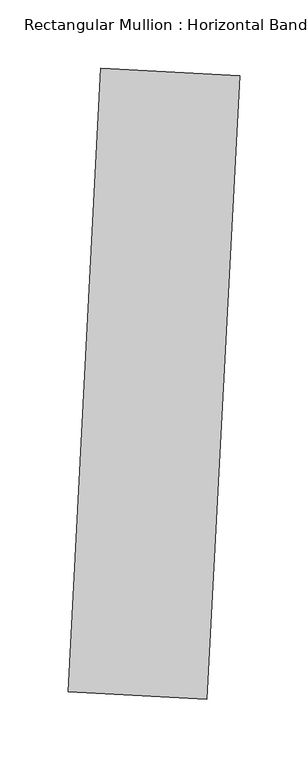
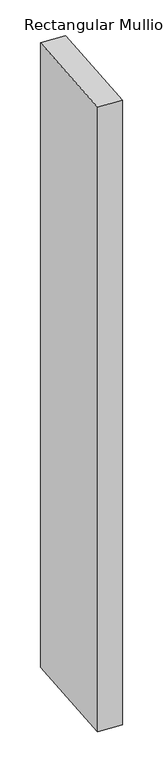
"""IFC4 building model written with IfcOpenShell, lengths in millimetres: member geometry, Rectangular Mullion : Horizontal Band."""

from ifc_helpers import new_model, si_unit, frame, origin, place, context, project, spatial, polyline, outline, extrude, source, transform, mapped, element, save


def rectangular_mullion_horizontal_band_1f6ee450(model_context):
    return source(origin(), model_context, "Body", "SweptSolid", [
        extrude(outline(polyline([(62.69438, 301.8280451), (38.7663808, -154.7453782), (-62.69438, -149.4280451), (-38.7663808, 307.1453782), (62.69438, 301.8280451)])), frame((0.0, 0.0, -2765.4069854), z_axis=(0.0, 0.0, 1.0), x_axis=(1.0, 0.0, 0.0)), (0.0, 0.0, 1.0), 2765.4069854),
    ])


if __name__ == "__main__":
    model = new_model("IFC4")
    model_context = context("Model", 3, world=origin())
    ifc_project = project(units=[si_unit("LENGTHUNIT", "METRE", prefix="MILLI")], contexts=[model_context])
    site = spatial("IfcSite", under=ifc_project)
    building = spatial("IfcBuilding", under=site)
    placement = place(None, origin())
    rectangular_mullion_horizontal_band_shape = rectangular_mullion_horizontal_band_1f6ee450(model_context)
    element("IfcMember", 1, ObjectType="Rectangular Mullion : Horizontal Band", at=placement, inside=building, context=model_context, shape_type="MappedRepresentation", body=[
        mapped(rectangular_mullion_horizontal_band_shape, transform((0.0, 0.0, 0.0), x_axis=(1.0, 0.0, 0.0), y_axis=(0.0, 1.0, 0.0), z_axis=(0.0, 0.0, 1.0))),
    ])
    save(model, "model.ifc")

# Revit data of these elements
# Type "Rectangular Mullion : Horizontal Band"
#   built-in parameter 1007351 = 0.25 (stored number, unit not read)
#   built-in parameter 1007304 = 1.5 (stored number, unit not read)
#   built-in parameter 1007301 = 0.166667 (stored number, unit not read)
#   built-in parameter 1007300 = 0.166667 (stored number, unit not read)
# Element 1 (IfcMember, "Rectangular Mullion : Horizontal Band")
#   Materials on its faces: "Aluminum"
# Materials
#   "Aluminum": class "Metal", colour RGB 247 247 247, transparency 0, Description = "Aluminum 6061", Cost = 0
